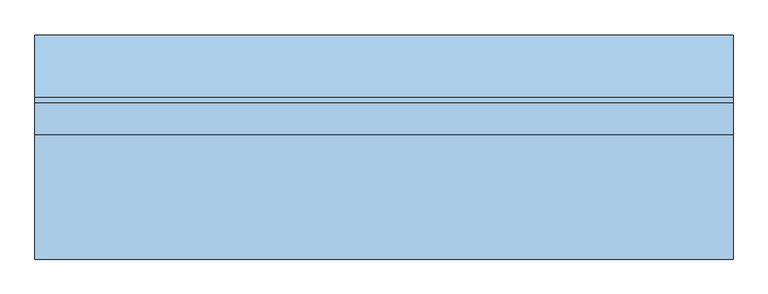
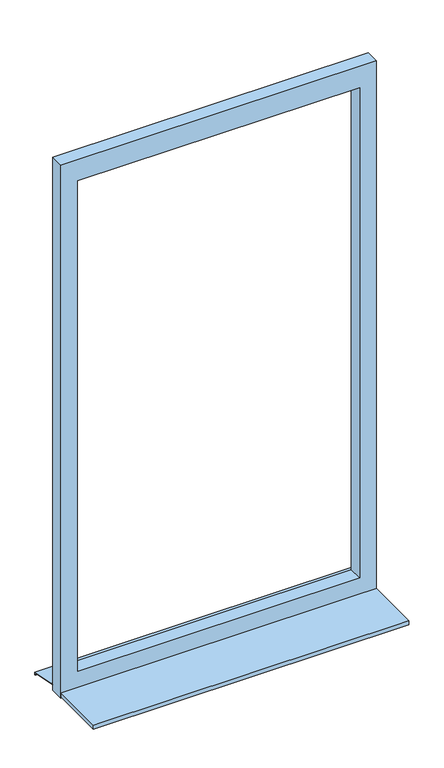
"""IFC4 building model written with IfcOpenShell, lengths in millimetres: window geometry, Fenster - Festverglasung : Feste Verglasung 1.25x2."""

from ifc_helpers import new_model, si_unit, frame, origin, place, context, project, spatial, polyline, outline, extrude, source, transform, mapped, element, save


def window_de583e7e(model_context):
    return source(origin(), model_context, "Body", "SweptSolid", [
        extrude(outline(polyline([(3000.0, 560.0), (3000.0, -560.0), (1000.0, -560.0), (1000.0, 560.0), (3000.0, 560.0)]), holes=[polyline([(2920.0, 500.0), (1080.0, 500.0), (1080.0, -500.0), (2920.0, -500.0), (2920.0, 500.0)])]), frame((0.0, 20.0, 0.0), z_axis=(0.0, 1.0, 0.0), x_axis=(0.0, 0.0, 1.0)), (0.0, 0.0, 1.0), 50.0),
        extrude(outline(polyline([(-560.0, -180.0), (-560.0, 20.0), (560.0, 20.0), (560.0, -180.0), (-560.0, -180.0)])), frame((0.0, 0.0, 1005.0), z_axis=(0.0, 0.0, 1.0), x_axis=(1.0, 0.0, 0.0)), (0.0, 0.0, 1.0), 15.0),
        extrude(outline(polyline([(80.0221543, 1020.0), (180.0, 1000.0), (180.0, 990.0), (178.0, 990.0), (178.0, 998.3604634), (79.8240723, 1018.0), (70.0, 1018.0), (70.0, 1020.0), (80.0221543, 1020.0)])), frame((-560.0, 0.0, 0.0), z_axis=(1.0, 0.0, 0.0), x_axis=(0.0, 1.0, 0.0)), (0.0, 0.0, 1.0), 1120.0),
    ])


if __name__ == "__main__":
    model = new_model("IFC4")
    model_context = context("Model", 3, world=origin())
    ifc_project = project(units=[si_unit("LENGTHUNIT", "METRE", prefix="MILLI")], contexts=[model_context])
    site = spatial("IfcSite", under=ifc_project)
    building = spatial("IfcBuilding", under=site)
    placement = place(None, origin())
    window_shape = window_de583e7e(model_context)
    element("IfcWindow", 1, ObjectType="Fenster - Festverglasung : Feste Verglasung 1.25x2", at=placement, inside=building, context=model_context, shape_type="MappedRepresentation", body=[
        mapped(window_shape, transform((0.0, 0.0, 0.0), x_axis=(1.0, 0.0, 0.0), y_axis=(0.0, 1.0, 0.0), z_axis=(0.0, 0.0, 1.0))),
    ])
    save(model, "model.ifc")

# Revit data of these elements
# Type "Fenster - Festverglasung : Feste Verglasung 1.25x2"
#   Type Mark = "54"
#   Operation = "SinglePanel"
#   Keynote = "16.05.01"
#   Visual Light Transmittance = 0.9
#   Solar Heat Gain Coefficient = 0.78
#   Rough Width = 1.120 m
#   Rough Height = 2.000 m
#   Heat Transfer Coefficient (U) = 3.6886 W/(m²·K)
#   Rahmentiefe = 0.050 m
#   Rahmenhöhe unten = 0.080 m
#   Höhe oberer  Rahmen = 0.080 m
#   Rahmenbreite = 0.060 m
#   Height = 2.000 m
#   Einbautiefe (von außen) [instance default] = 0.080 m
#   Width = 1.120 m
#   Wall Closure = 2
#   Bild [instance default] = none
#   Glas [instance default] = none
#   Innere Fensterbank [instance default] = none
#   Äußere Fensterbank [instance default] = none
#   Construction Type Id = ""
#   Analytic Construction = (empty or 0)
# Element 1 (IfcWindow, "Fenster - Festverglasung : Feste Verglasung 1.25x2")
#   Materials on its faces: "Kunststoff - Weiß", "Holz - Birke"
# Materials
#   "Kunststoff - Weiß": class "Kunststoff", colour RGB 249 249 249, transparency 0, Cost = 0
#   "Holz - Birke": class "Holz", colour RGB 213 164 103, transparency 0, Cost = 0
